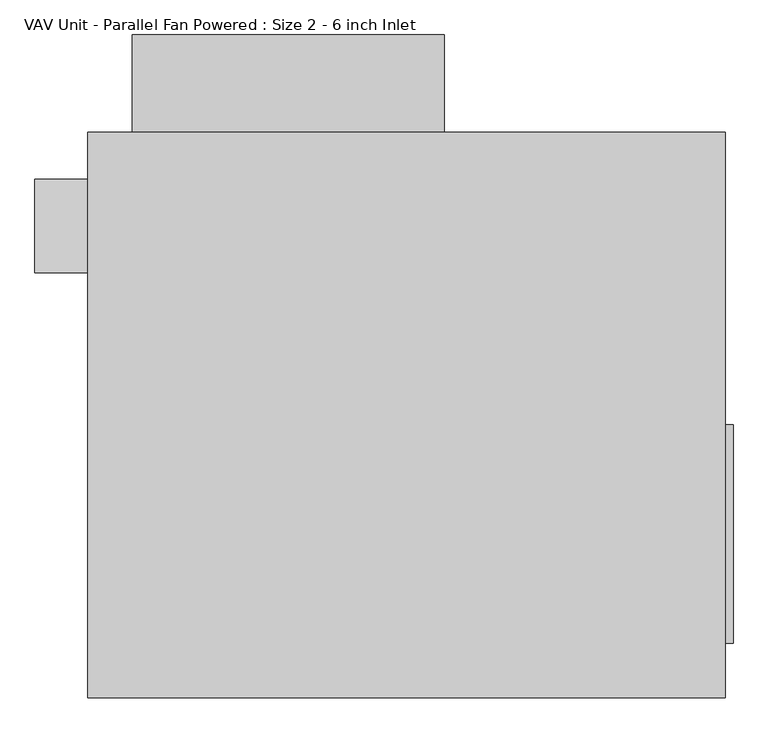
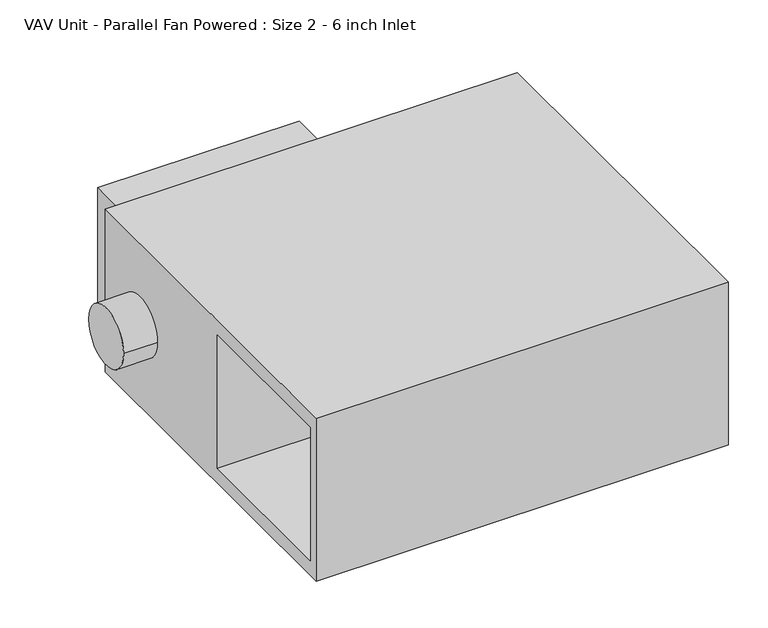
"""IFC4 building model written with IfcOpenShell, lengths in millimetres: proxy geometry, VAV Unit - Parallel Fan Powered : Size 2 - 6 inch Inlet."""

from ifc_helpers import new_model, si_unit, point, frame, frame_2d, origin, place, context, project, spatial, polyline, circle_curve, trimmed, segment, composite_curve, outline, extrude, faceted_brep, source, transform, mapped, element, save


def vav_unit_parallel_fan_powered_size_2_6_inch_inlet_6222e6d5(model_context):
    return source(origin(), model_context, "Body", "SolidModel", [
        extrude(outline(polyline([(531.8125, -15.875), (531.8125, -371.475), (519.1125, -371.475), (519.1125, -15.875), (531.8125, -15.875)])), frame((0.0, 0.0, -139.7), z_axis=(0.0, 0.0, 1.0), x_axis=(1.0, 0.0, 0.0)), (0.0, 0.0, 1.0), 279.4),
        extrude(outline(polyline([(61.9125, 460.375), (-446.0875, 460.375), (-446.0875, 619.125), (61.9125, 619.125), (61.9125, 460.375)])), frame((0.0, 0.0, -152.4), z_axis=(0.0, 0.0, 1.0), x_axis=(1.0, 0.0, 0.0)), (0.0, 0.0, 1.0), 304.8),
        extrude(outline(composite_curve([segment(trimmed(circle_curve(frame_2d((307.975, 0.0)), 76.2), [point((231.775, 0.0))], [point((384.175, 0.0))], False, "CARTESIAN"), True, "CONTINUOUS"), segment(trimmed(circle_curve(frame_2d((307.975, 0.0)), 76.2), [point((384.175, 0.0))], [point((231.775, 0.0))], False, "CARTESIAN"), True, "CONTINUOUS")], self_intersect=False)), frame((-604.8375, 0.0, 0.0), z_axis=(1.0, 0.0, 0.0), x_axis=(0.0, 1.0, 0.0)), (0.0, 0.0, 1.0), 85.725),
        faceted_brep([(519.1125, 460.375, 217.4875), (-519.1125, 460.375, 217.4875), (-519.1125, -460.375, 217.4875), (519.1125, -460.375, 217.4875), (519.1125, 460.375, -217.4875), (519.1125, -460.375, -217.4875), (-519.1125, -460.375, -217.4875), (-519.1125, 460.375, -217.4875), (-519.1125, -434.975, 177.8), (-519.1125, -434.975, -177.8), (-519.1125, -28.575, -177.8), (-519.1125, -28.575, 177.8), (0.0, -434.975, 177.8), (0.0, -28.575, 177.8), (0.0, -28.575, -177.8), (0.0, -434.975, -177.8)], [[[0, 1, 2, 3]], [[4, 5, 6, 7]], [[1, 0, 4, 7]], [[2, 1, 7, 6], [8, 9, 10, 11]], [[3, 2, 6, 5]], [[0, 3, 5, 4]], [[12, 13, 14, 15]], [[12, 15, 9, 8]], [[15, 14, 10, 9]], [[14, 13, 11, 10]], [[13, 12, 8, 11]]]),
    ])


if __name__ == "__main__":
    model = new_model("IFC4")
    model_context = context("Model", 3, world=origin())
    ifc_project = project(units=[si_unit("LENGTHUNIT", "METRE", prefix="MILLI")], contexts=[model_context])
    site = spatial("IfcSite", under=ifc_project)
    building = spatial("IfcBuilding", under=site)
    placement = place(None, origin())
    vav_unit_parallel_fan_powered_size_2_6_inch_inlet_shape = vav_unit_parallel_fan_powered_size_2_6_inch_inlet_6222e6d5(model_context)
    element("IfcBuildingElementProxy", 1, Name="VAV Unit - Parallel Fan Powered : Size 2 - 6 inch Inlet", ObjectType="VAV Unit - Parallel Fan Powered : Size 2 - 6 inch Inlet", at=placement, inside=building, context=model_context, shape_type="MappedRepresentation", body=[
        mapped(vav_unit_parallel_fan_powered_size_2_6_inch_inlet_shape, transform((0.0, 0.0, 0.0), x_axis=(1.0, 0.0, 0.0), y_axis=(0.0, 1.0, 0.0), z_axis=(0.0, 0.0, 1.0))),
    ])
    save(model, "model.ifc")

# Revit data of these elements
# Type "VAV Unit - Parallel Fan Powered : Size 2 - 6 inch Inlet"
#   Width2 = 1' - 2"
#   Voltage = 120 V
#   UnitWidth = 3' - 4 7/8"
#   UnitHeight = 3' - 0 1/4"
#   UnitDepth = 1' - 5 1/8"
#   SupplyConnectorWidth = 1' - 2"
#   SupplyConnectorVerticalOffset = 0' - 2 1/8"
#   SupplyConnectorLength = 0' - 0 1/2"
#   SupplyConnectorHorizontalOffset = 0' - 3 1/2"
#   SupplyConnectorDepth = 0' - 11"
#   SupplyAirConnectorCenterOffset = 0' - 10 1/2"
#   PrimaryToSupplyRatio [instance default] = 0.2
#   PrimaryAirOffset = 0' - 6"
#   PrimaryAirFlow [instance default] = 100 CFM
#   PrimaryAirConnectorVerticalOffset = 0' - 8 9/16"
#   PrimaryAirConnectorRadius = 0' - 3"
#   PrimaryAirConnectorLength = 0' - 3 3/8"
#   PrimaryAirConnectorDiameter = 0' - 6"
#   PrimaryAirConnectorCenterOffset = 0' - 6"
#   Pressure Drop [instance default] = 0.04 in-wg
#   InducedAirInletWidth = 1' - 4"
#   InducedAirInletDepth = 1' - 2"
#   InducedAirConnectorHorizontalOffset = 0' - 1"
#   InducedAirConnectorCenterOffset = 0' - 9"
#   Height2 = 0' - 11"
#   ElectricalConnectionBoxWidth = 1' - 8"
#   ElectricalConnectionBoxOffset = 0' - 2 7/8"
#   ElectricalConnectionBoxHeight = 0' - 6 1/4"
#   ElectricalConnectionBoxDepth = 1' - 0"
#   SupplyAirFlow [instance default] = 500 CFM
#   Apparent Load = 181 VA
#   SupplyAirConnectorIndex = 2
#   PrimaryAirConnectorIndex = 1
#   Number of Poles = 1
#   InducedAirConnectorIndex = 3
#   VAV Material = none
#   Load Classification = Cooling
#   Default Elevation = 0
#   Assembly Code = ""
